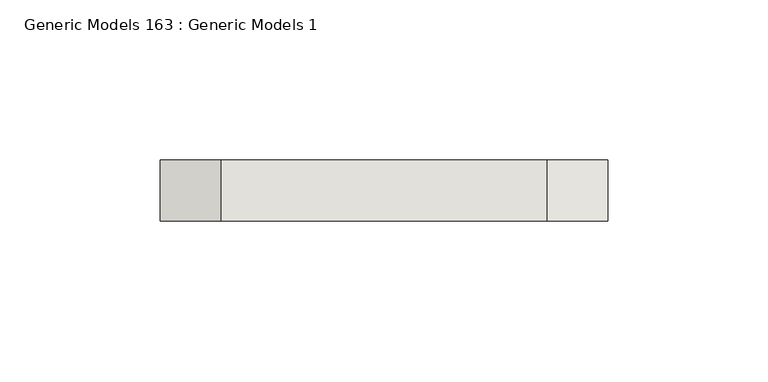
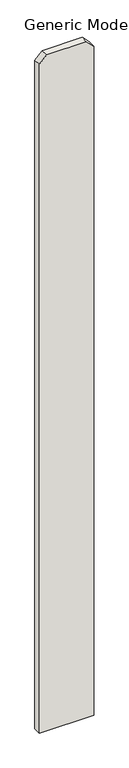
"""IFC4 building model written with IfcOpenShell, lengths in millimetres: wall geometry, Generic Models 163 : Generic Models 1."""

from ifc_helpers import new_model, si_unit, frame, origin, place, context, project, spatial, polyline, outline, extrude, source, transform, mapped, element, save


def generic_models_163_generic_models_1_77b09895(model_context):
    return source(origin(), model_context, "Body", "SweptSolid", [
        extrude(outline(polyline([(76.2, 323823.0125), (1885.95, 323823.0125), (1905.0, 323803.9625), (1905.0, 323702.3625), (1885.95, 323683.3125), (76.2, 323683.3125), (76.2, 323823.0125)])), frame((0.0, 547.6875, 0.0), z_axis=(0.0, 1.0, 0.0), x_axis=(0.0, 0.0, 1.0)), (0.0, 0.0, 1.0), 19.05),
    ])


if __name__ == "__main__":
    model = new_model("IFC4")
    model_context = context("Model", 3, world=origin())
    ifc_project = project(units=[si_unit("LENGTHUNIT", "METRE", prefix="MILLI")], contexts=[model_context])
    site = spatial("IfcSite", under=ifc_project)
    building = spatial("IfcBuilding", under=site)
    placement = place(None, origin())
    generic_models_163_generic_models_1_shape = generic_models_163_generic_models_1_77b09895(model_context)
    element("IfcWall", 1, ObjectType="Generic Models 163 : Generic Models 1", at=placement, inside=building, context=model_context, shape_type="MappedRepresentation", body=[
        mapped(generic_models_163_generic_models_1_shape, transform((0.0, 0.0, 0.0), x_axis=(1.0, 0.0, 0.0), y_axis=(0.0, 1.0, 0.0), z_axis=(0.0, 0.0, 1.0))),
    ])
    save(model, "model.ifc")

# Revit data of these elements
# Element 1 (IfcWall, "Generic Models 163 : Generic Models 1")
#   Materials on its faces: "VERTICAL 1X6 CEDAR PLANKS W/ CLEAR WOOD SEALER"
# Materials
#   "VERTICAL 1X6 CEDAR PLANKS W/ CLEAR WOOD SEALER": class "Wood", colour RGB 234 198 147, transparency 0, Description = "Pinus Echinata", Cost = 0
